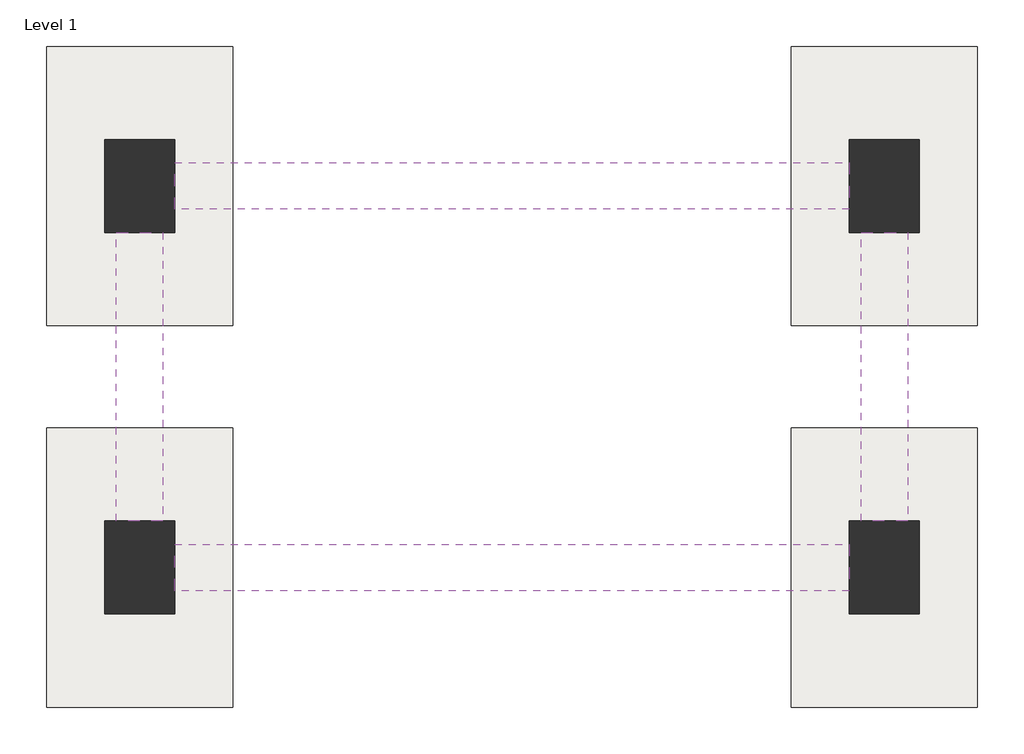
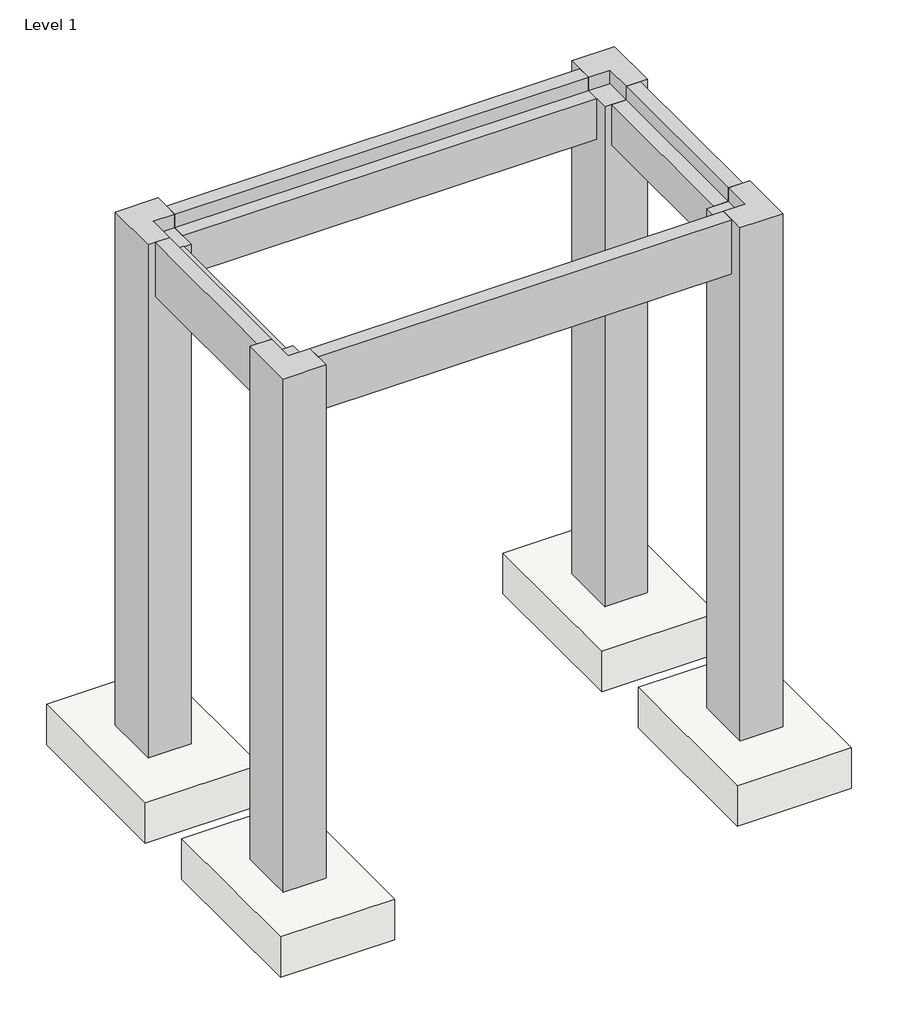
# One storey: 4 beams, 4 columns, 4 slabs.
"""IFC4 building model written with IfcOpenShell, lengths in millimetres."""

import ifcopenshell
import ifcopenshell.guid

model = None  # the IFC model being written
_history = None  # IfcOwnerHistory: only IFC2X3 demands one
_inside = {}  # id of a spatial element -> (the spatial element, [elements in it])
_under = {}  # id of a project, library or spatial element -> (it, [spatial elements below it])
_declared = {}  # id of a project -> (the project, [libraries it declares])
_typed = {}  # id of a type object -> (the type object, [elements of that type])
_made_of = {}  # id of a material, layer set ... -> (it, [elements and type objects made of it])


def new_model(schema):
    """Start an empty IFC model of exactly this schema.

    Asked for "IFC4X3", IfcOpenShell would pick the latest addendum, in which some entities
    have other attributes; the version numbers below select the first issue.
    IFC2X3 requires an IfcOwnerHistory on every rooted entity: one is made here for all.
    """
    global model, _history
    if schema == "IFC4X3":
        model = ifcopenshell.file(schema_version=(4, 3, 0, 0))
    else:
        model = ifcopenshell.file(schema=schema)
    _inside.clear()
    _under.clear()
    _declared.clear()
    _typed.clear()
    _made_of.clear()
    _history = None
    if model.schema == "IFC2X3":
        org = make("IfcOrganization", Name="unknown")
        user = make(
            "IfcPersonAndOrganization",
            ThePerson=make("IfcPerson", FamilyName="unknown"),
            TheOrganization=org,
        )
        app = make(
            "IfcApplication",
            ApplicationDeveloper=org,
            Version="unknown",
            ApplicationFullName="unknown",
            ApplicationIdentifier="unknown",
        )
        _history = make(
            "IfcOwnerHistory",
            OwningUser=user,
            OwningApplication=app,
            ChangeAction="ADDED",
            CreationDate=0,
        )
    return model


def make(cls, **values):
    """One entity of the class cls with the attributes given. An attribute that is None is left unset."""
    return model.create_entity(
        cls, **{name: value for name, value in values.items() if value is not None}
    )


def rooted(cls, **values):
    """An entity with a GlobalId (a new one), such as an element, a storey or a relation."""
    return make(cls, GlobalId=ifcopenshell.guid.new(), OwnerHistory=_history, **values)


def si_unit(unit_type, name, prefix=None):
    """IfcSIUnit, for example si_unit("LENGTHUNIT", "METRE", prefix="MILLI")."""
    return make("IfcSIUnit", UnitType=unit_type, Prefix=prefix, Name=name)


def assignment(units):
    """IfcUnitAssignment: the units of a project."""
    return None if units is None else make("IfcUnitAssignment", Units=units)


def point(xyz):
    """IfcCartesianPoint."""
    return None if xyz is None else make("IfcCartesianPoint", Coordinates=xyz)


def direction(xyz):
    """IfcDirection."""
    return None if xyz is None else make("IfcDirection", DirectionRatios=xyz)


def frame(location, z_axis=None, x_axis=None):
    """IfcAxis2Placement3D, a coordinate frame: its origin and axes. An axis left out is left unset."""
    return make(
        "IfcAxis2Placement3D",
        Location=point(location),
        Axis=direction(z_axis),
        RefDirection=direction(x_axis),
    )


def origin():
    """The frame at (0, 0, 0) with its axes left unset."""
    return frame((0.0, 0.0, 0.0))


def place(relative_to, where):
    """IfcLocalPlacement: puts the frame where relative to a parent placement (None: the world)."""
    return make(
        "IfcLocalPlacement", PlacementRelTo=relative_to, RelativePlacement=where
    )


def context(
    kind, dimensions, precision=None, world=None, true_north=None, identifier=None
):
    """IfcGeometricRepresentationContext, for example the 3D "Model" context."""
    return make(
        "IfcGeometricRepresentationContext",
        ContextIdentifier=identifier,
        ContextType=kind,
        CoordinateSpaceDimension=dimensions,
        Precision=precision,
        WorldCoordinateSystem=world,
        TrueNorth=true_north,
    )


def project(units=None, contexts=None):
    """IfcProject with its units and contexts."""
    return rooted(
        "IfcProject",
        Name="project",
        RepresentationContexts=contexts,
        UnitsInContext=assignment(units),
    )


def spatial(cls, under=None, at=None, **own):
    """A site, building, storey or space (cls), placed at a placement, below another one or the project."""
    s = rooted(cls, ObjectPlacement=at, **own)
    if under is not None:
        _under.setdefault(under.id(), (under, []))[1].append(s)
    return s


def polyline(points):
    """IfcPolyline through the points."""
    return make("IfcPolyline", Points=[point(p) for p in points])


def outline(outer, holes=None, kind="AREA"):
    """IfcArbitraryClosedProfileDef: a profile drawn as a closed curve; with holes, ...WithVoids."""
    if holes is None:
        return make("IfcArbitraryClosedProfileDef", ProfileType=kind, OuterCurve=outer)
    return make(
        "IfcArbitraryProfileDefWithVoids",
        ProfileType=kind,
        OuterCurve=outer,
        InnerCurves=holes,
    )


def extrude(swept, where, along, depth):
    """IfcExtrudedAreaSolid: the profile swept, set in the frame where, extruded along a direction by depth."""
    return make(
        "IfcExtrudedAreaSolid",
        SweptArea=swept,
        Position=where,
        ExtrudedDirection=direction(along),
        Depth=depth,
    )


def faces_of(points, faces, orient=None, outer=None):
    """IfcFace entities. A face is a list of loops; a loop is a list of indices into points, from 0.

    orient and outer hold one flag for each loop. By default every Orientation is true, the
    first loop of a face is its IfcFaceOuterBound and the others are IfcFaceBound.
    """
    made = []
    for i, loops in enumerate(faces):
        bounds = []
        for j, loop in enumerate(loops):
            is_outer = j == 0 if outer is None else outer[i][j]
            bounds.append(
                make(
                    "IfcFaceOuterBound" if is_outer else "IfcFaceBound",
                    Bound=make("IfcPolyLoop", Polygon=[points[k] for k in loop]),
                    Orientation=True if orient is None else orient[i][j],
                )
            )
        made.append(make("IfcFace", Bounds=bounds))
    return made


def faceted_brep(points, faces, orient=None, outer=None, voids=None):
    """IfcFacetedBrep: a solid bounded by flat faces; with voids (closed shells), ...WithVoids."""
    shared = [point(p) for p in points]
    hull = make("IfcClosedShell", CfsFaces=faces_of(shared, faces, orient, outer))
    if voids is None:
        return make("IfcFacetedBrep", Outer=hull)
    return make(
        "IfcFacetedBrepWithVoids",
        Outer=hull,
        Voids=[
            make(cls, CfsFaces=faces_of(shared, fs, o, b)) for cls, fs, o, b in voids
        ],
    )


def shape(context_of_items, identifier, shape_type, items):
    """IfcShapeRepresentation: the items that make up one representation, for example the "Body"."""
    return make(
        "IfcShapeRepresentation",
        ContextOfItems=context_of_items,
        RepresentationIdentifier=identifier,
        RepresentationType=shape_type,
        Items=items,
    )


def source(mapping_origin, context_of_items, identifier, shape_type, items):
    """IfcRepresentationMap: a shape defined once, which mapped items show again and again."""
    return make(
        "IfcRepresentationMap",
        MappingOrigin=mapping_origin,
        MappedRepresentation=shape(context_of_items, identifier, shape_type, items),
    )


def transform(
    local_origin,
    x_axis=None,
    y_axis=None,
    z_axis=None,
    scale=None,
    scale2=None,
    scale3=None,
    uniform=True,
):
    """IfcCartesianTransformationOperator3D, or its non-uniform kind. x_axis, y_axis, z_axis: its Axis1, 2, 3."""
    if uniform:
        return make(
            "IfcCartesianTransformationOperator3D",
            Axis1=direction(x_axis),
            Axis2=direction(y_axis),
            LocalOrigin=point(local_origin),
            Scale=scale,
            Axis3=direction(z_axis),
        )
    return make(
        "IfcCartesianTransformationOperator3DnonUniform",
        Axis1=direction(x_axis),
        Axis2=direction(y_axis),
        LocalOrigin=point(local_origin),
        Scale=scale,
        Axis3=direction(z_axis),
        Scale2=scale2,
        Scale3=scale3,
    )


def mapped(mapping_source, mapping_target):
    """IfcMappedItem: shows the shape of a source again, moved by a transform."""
    return make(
        "IfcMappedItem", MappingSource=mapping_source, MappingTarget=mapping_target
    )


def made_of(thing, what):
    """Note that an element or type object is made of a material, layer set ...; save() writes the relation."""
    if what is not None:
        _made_of.setdefault(what.id(), (what, []))[1].append(thing)
    return thing


def element(
    cls,
    number,
    at=None,
    inside=None,
    cuts=None,
    type_object=None,
    material=None,
    context=None,
    identifier="Body",
    shape_type=None,
    held_by="IfcProductDefinitionShape",
    body=None,
    shapes=None,
    **own,
):
    """One element of the class cls, such as IfcWall. Its Tag is "e" and its number.

    at: its placement. inside: the storey or other place that contains it. cuts: it is an
    opening in that element (IfcRelVoidsElement). A single representation is given by context,
    identifier, shape_type and body (its items); several are given by shapes. held_by: the class
    of the entity that holds the representations. save() writes the other relations.
    """
    e = rooted(cls, Tag="e%d" % number, ObjectPlacement=at, **own)
    if body is not None:
        shapes = [shape(context, identifier, shape_type, body)]
    if shapes is not None:
        e.Representation = make(held_by, Representations=shapes)
    if inside is not None:
        _inside.setdefault(inside.id(), (inside, []))[1].append(e)
    if cuts is not None:
        rooted(
            "IfcRelVoidsElement", RelatingBuildingElement=cuts, RelatedOpeningElement=e
        )
    if type_object is not None:
        _typed.setdefault(type_object.id(), (type_object, []))[1].append(e)
    return made_of(e, material)


def aggregate(whole, parts):
    """IfcRelAggregates: a whole, such as a stair, and the parts it consists of."""
    return rooted("IfcRelAggregates", RelatingObject=whole, RelatedObjects=parts)


def save(model, path):
    """Write the relations noted so far, then the file.

    IfcRelAggregates (storeys below a building ...), IfcRelContainedInSpatialStructure (elements
    in a storey), IfcRelDefinesByType, IfcRelAssociatesMaterial and IfcRelDeclares: one each for
    every whole, place, type object, material and project.
    """
    for whole, parts in _under.values():
        aggregate(whole, parts)
    for where, things in _inside.values():
        rooted(
            "IfcRelContainedInSpatialStructure",
            RelatedElements=things,
            RelatingStructure=where,
        )
    for kind, things in _typed.values():
        rooted("IfcRelDefinesByType", RelatedObjects=things, RelatingType=kind)
    for what, things in _made_of.values():
        rooted("IfcRelAssociatesMaterial", RelatedObjects=things, RelatingMaterial=what)
    for by, libraries in _declared.values():
        rooted("IfcRelDeclares", RelatingContext=by, RelatedDefinitions=libraries)
    model.write(path)


def slab_5ba74754(model_context):
    return source(origin(), model_context, "Body", "SweptSolid", [
        extrude(outline(polyline([(609.6, 914.4), (609.6, -914.4), (-609.6, -914.4), (-609.6, 914.4), (609.6, 914.4)])), frame((0.0, 0.0, -457.2), z_axis=(0.0, 0.0, 1.0), x_axis=(1.0, 0.0, 0.0)), (0.0, 0.0, 1.0), 457.2),
    ])


model = new_model("IFC4")

# Units and contexts
model_context = context("Model", 3, world=origin())
ifc_project = project(units=[si_unit("LENGTHUNIT", "METRE", prefix="MILLI")], contexts=[model_context])

# Site, building, storey
site = spatial("IfcSite", under=ifc_project)
building = spatial("IfcBuilding", under=site)
storey = spatial("IfcBuildingStorey", under=building, Name="Level 1", Elevation=0.0)

# Beams
placement = place(None, origin())
element("IfcBeam", 1, ObjectType="Concrete-Rectangular Beam : 12 x 24", at=placement, inside=storey, context=model_context, shape_type="SweptSolid", body=[
    extrude(outline(polyline([(6090.8323826, 2438.4), (5786.0323826, 2438.4), (5786.0323826, 2895.6), (5938.4323826, 2895.6), (5938.4323826, 3048.0), (6090.8323826, 3048.0), (6090.8323826, 2438.4)])), frame((-11045.0800525, 0.0, 0.0), z_axis=(1.0, 0.0, 0.0), x_axis=(0.0, 1.0, 0.0)), (0.0, 0.0, 1.0), 4419.6),
])
element("IfcBeam", 2, ObjectType="Concrete-Rectangular Beam : 12 x 24", at=placement, inside=storey, context=model_context, shape_type="SweptSolid", body=[
    extrude(outline(polyline([(3286.0323826, 2438.4), (3286.0323826, 3048.0), (3438.4323826, 3048.0), (3438.4323826, 2895.6), (3590.8323826, 2895.6), (3590.8323826, 2438.4), (3286.0323826, 2438.4)])), frame((-11045.0800525, 0.0, 0.0), z_axis=(1.0, 0.0, 0.0), x_axis=(0.0, 1.0, 0.0)), (0.0, 0.0, 1.0), 4419.6),
])
element("IfcBeam", 3, ObjectType="Concrete-Rectangular Beam : 12 x 24", at=placement, inside=storey, context=model_context, shape_type="SweptSolid", body=[
    extrude(outline(polyline([(2438.4, -6549.2800525), (2438.4, -6244.4800525), (3048.0, -6244.4800525), (3048.0, -6396.8800525), (2895.6, -6396.8800525), (2895.6, -6549.2800525), (2438.4, -6549.2800525)])), frame((0.0, 3743.2323826, 0.0), z_axis=(0.0, 1.0, 0.0), x_axis=(0.0, 0.0, 1.0)), (0.0, 0.0, 1.0), 1890.4),
])
element("IfcBeam", 4, ObjectType="Concrete-Rectangular Beam : 12 x 24", at=placement, inside=storey, context=model_context, shape_type="SweptSolid", body=[
    extrude(outline(polyline([(2438.4, -11426.0800525), (2438.4, -11121.2800525), (2895.6, -11121.2800525), (2895.6, -11273.6800525), (3048.0, -11273.6800525), (3048.0, -11426.0800525), (2438.4, -11426.0800525)])), frame((0.0, 3743.2323826, 0.0), z_axis=(0.0, 1.0, 0.0), x_axis=(0.0, 0.0, 1.0)), (0.0, 0.0, 1.0), 1890.4),
])

# Columns
element("IfcColumn", 5, ObjectType="Concrete-Rectangular-Column : 18 x 24", at=placement, inside=storey, context=model_context, shape_type="Brep", body=[
    faceted_brep([(-11045.0800525, 6243.2323826, 3048.0), (-11502.2800525, 6243.2323826, 3048.0), (-11502.2800525, 5633.6323826, 3048.0), (-11273.6800525, 5633.6323826, 3048.0), (-11273.6800525, 5938.4323826, 3048.0), (-11045.0800525, 5938.4323826, 3048.0), (-11045.0800525, 6243.2323826, -2743.2), (-11045.0800525, 5633.6323826, -2743.2), (-11502.2800525, 5633.6323826, -2743.2), (-11502.2800525, 6243.2323826, -2743.2), (-11045.0800525, 5633.6323826, 2895.6), (-11273.6800525, 5633.6323826, 2895.6), (-11045.0800525, 5938.4323826, 2895.6), (-11273.6800525, 5938.4323826, 2895.6)], [[[0, 1, 2, 3, 4, 5]], [[6, 7, 8, 9]], [[1, 0, 6, 9]], [[2, 1, 9, 8]], [[8, 7, 10, 11, 3, 2]], [[7, 6, 0, 5, 12, 10]], [[12, 13, 11, 10]], [[13, 4, 3, 11]], [[4, 13, 12, 5]]]),
])
element("IfcColumn", 6, ObjectType="Concrete-Rectangular-Column : 18 x 24", at=placement, inside=storey, context=model_context, shape_type="Brep", body=[
    faceted_brep([(-6168.2800525, 6243.2323826, 3048.0), (-6625.4800525, 6243.2323826, 3048.0), (-6625.4800525, 5938.4323826, 3048.0), (-6396.8800525, 5938.4323826, 3048.0), (-6396.8800525, 5633.6323826, 3048.0), (-6168.2800525, 5633.6323826, 3048.0), (-6168.2800525, 6243.2323826, -2743.2), (-6168.2800525, 5633.6323826, -2743.2), (-6625.4800525, 5633.6323826, -2743.2), (-6625.4800525, 6243.2323826, -2743.2), (-6625.4800525, 5633.6323826, 2895.6), (-6625.4800525, 5938.4323826, 2895.6), (-6396.8800525, 5633.6323826, 2895.6), (-6396.8800525, 5938.4323826, 2895.6)], [[[0, 1, 2, 3, 4, 5]], [[6, 7, 8, 9]], [[1, 0, 6, 9]], [[9, 8, 10, 11, 2, 1]], [[8, 7, 5, 4, 12, 10]], [[0, 5, 7, 6]], [[13, 11, 10, 12]], [[3, 13, 12, 4]], [[13, 3, 2, 11]]]),
])
element("IfcColumn", 7, ObjectType="Concrete-Rectangular-Column : 18 x 24", at=placement, inside=storey, context=model_context, shape_type="Brep", body=[
    faceted_brep([(-11502.2800525, 3743.2323826, 3048.0), (-11502.2800525, 3133.6323826, 3048.0), (-11045.0800525, 3133.6323826, 3048.0), (-11045.0800525, 3438.4323826, 3048.0), (-11273.6800525, 3438.4323826, 3048.0), (-11273.6800525, 3743.2323826, 3048.0), (-11045.0800525, 3743.2323826, -2743.2), (-11045.0800525, 3133.6323826, -2743.2), (-11502.2800525, 3133.6323826, -2743.2), (-11502.2800525, 3743.2323826, -2743.2), (-11273.6800525, 3743.2323826, 2895.6), (-11045.0800525, 3743.2323826, 2895.6), (-11045.0800525, 3438.4323826, 2895.6), (-11273.6800525, 3438.4323826, 2895.6)], [[[0, 1, 2, 3, 4, 5]], [[6, 7, 8, 9]], [[6, 9, 0, 5, 10, 11]], [[1, 0, 9, 8]], [[2, 1, 8, 7]], [[7, 6, 11, 12, 3, 2]], [[10, 13, 12, 11]], [[13, 4, 3, 12]], [[4, 13, 10, 5]]]),
])
element("IfcColumn", 8, ObjectType="Concrete-Rectangular-Column : 18 x 24", at=placement, inside=storey, context=model_context, shape_type="Brep", body=[
    faceted_brep([(-6625.4800525, 3133.6323826, 3048.0), (-6168.2800525, 3133.6323826, 3048.0), (-6168.2800525, 3743.2323826, 3048.0), (-6396.8800525, 3743.2323826, 3048.0), (-6396.8800525, 3438.4323826, 3048.0), (-6625.4800525, 3438.4323826, 3048.0), (-6168.2800525, 3743.2323826, -2743.2), (-6168.2800525, 3133.6323826, -2743.2), (-6625.4800525, 3133.6323826, -2743.2), (-6625.4800525, 3743.2323826, -2743.2), (-6625.4800525, 3743.2323826, 2895.6), (-6396.8800525, 3743.2323826, 2895.6), (-6625.4800525, 3438.4323826, 2895.6), (-6396.8800525, 3438.4323826, 2895.6)], [[[0, 1, 2, 3, 4, 5]], [[6, 7, 8, 9]], [[6, 9, 10, 11, 3, 2]], [[9, 8, 0, 5, 12, 10]], [[1, 0, 8, 7]], [[2, 1, 7, 6]], [[12, 13, 11, 10]], [[13, 4, 3, 11]], [[4, 13, 12, 5]]]),
])

# Slabs
slab_shape = slab_5ba74754(model_context)
element("IfcSlab", 9, ObjectType="Footing-Rectangular : 72\" x 48\" x 18\"", at=placement, inside=storey, context=model_context, shape_type="MappedRepresentation", body=[
    mapped(slab_shape, transform((-11273.6800525, 5938.4323826, -2743.2), x_axis=(1.0, 0.0, 0.0), y_axis=(0.0, 1.0, 0.0), z_axis=(0.0, 0.0, 1.0))),
])
element("IfcSlab", 10, ObjectType="Footing-Rectangular : 72\" x 48\" x 18\"", at=placement, inside=storey, context=model_context, shape_type="MappedRepresentation", body=[
    mapped(slab_shape, transform((-6396.8800525, 5938.4323826, -2743.2), x_axis=(1.0, 0.0, 0.0), y_axis=(0.0, 1.0, 0.0), z_axis=(0.0, 0.0, 1.0))),
])
element("IfcSlab", 11, ObjectType="Footing-Rectangular : 72\" x 48\" x 18\"", at=placement, inside=storey, context=model_context, shape_type="MappedRepresentation", body=[
    mapped(slab_shape, transform((-11273.6800525, 3438.4323826, -2743.2), x_axis=(1.0, 0.0, 0.0), y_axis=(0.0, 1.0, 0.0), z_axis=(0.0, 0.0, 1.0))),
])
element("IfcSlab", 12, ObjectType="Footing-Rectangular : 72\" x 48\" x 18\"", at=placement, inside=storey, context=model_context, shape_type="MappedRepresentation", body=[
    mapped(slab_shape, transform((-6396.8800525, 3438.4323826, -2743.2), x_axis=(1.0, 0.0, 0.0), y_axis=(0.0, 1.0, 0.0), z_axis=(0.0, 0.0, 1.0))),
])

save(model, "model.ifc")

# Revit data of these elements
# Project information
#   Project Issue Date = "Issue Date"
#   Project Status = "Project Status"
#   Client Name = "Owner"
#   Project Address = "Enter address here"
#   Project Name = "Project Name"
#   Project Number = "Project Number"
# Grids (mm)
#   "1": line (9019.216, 5938.432) -> (-21563.036, 5938.432)
#   "2": line (-11273.68, -9686.145) -> (-11273.68, 17085.235)
#   "3": line (-6396.88, 17085.235) -> (-6396.88, -9686.145)
#   "4": line (3059.851, 3438.432) -> (-21143.609, 3438.432)
# Type "Concrete-Rectangular Beam : 12 x 24"
#   Assembly Code = "B10"
#   Length [instance default] = 1.524 m
#   b = 0.3048 m
#   h = 0.6096 m
#   Structural Material [instance default] = Concrete - Cast-in-Place Concrete
# Type "Concrete-Rectangular-Column : 18 x 24"
#   Assembly Code = "B10"
#   b = 0.4572 m
#   h = 0.6096 m
#   Structural Material [instance default] = Concrete - Cast-in-Place Concrete
# Type "Footing-Rectangular : 72\" x 48\" x 18\""
#   Assembly Code = "A1010100"
#   Width = 1.2192 m
#   Length = 1.8288 m
#   Thickness = 0.4572 m
#   Structural Material [instance default] = Concrete - Cast-in-Place Concrete
# Elements 1, 2, 3, 4 (IfcBeam, "Concrete-Rectangular Beam : 12 x 24")
#   Comments = ""
#   Structural Material = Concrete - Cast-in-Place Concrete
#   Phase Created = New Construction
#   Materials on its faces: "Concrete - Cast-in-Place Concrete"
# Elements 5, 6, 7, 8 (IfcColumn, "Concrete-Rectangular-Column : 18 x 24")
#   Structural Material = Concrete - Cast-in-Place Concrete
#   Phase Created = New Construction
#   Materials on its faces: "Concrete - Cast-in-Place Concrete"
# Element 9 (IfcSlab, "Footing-Rectangular : 72\" x 48\" x 18\"")
#   Structural Material = Concrete - Cast-in-Place Concrete
#   Phase Created = New Construction
#   Materials on its faces: "Concrete - Cast-in-Place Concrete"
# Elements 10, 11, 12 (IfcSlab, "Footing-Rectangular : 72\" x 48\" x 18\"")
#   Comments = ""
#   Structural Material = Concrete - Cast-in-Place Concrete
#   Phase Created = New Construction
#   Materials on its faces: "Concrete - Cast-in-Place Concrete"
# Materials
#   "Concrete - Cast-in-Place Concrete": class "Concrete", colour RGB 192 192 192, transparency 0
